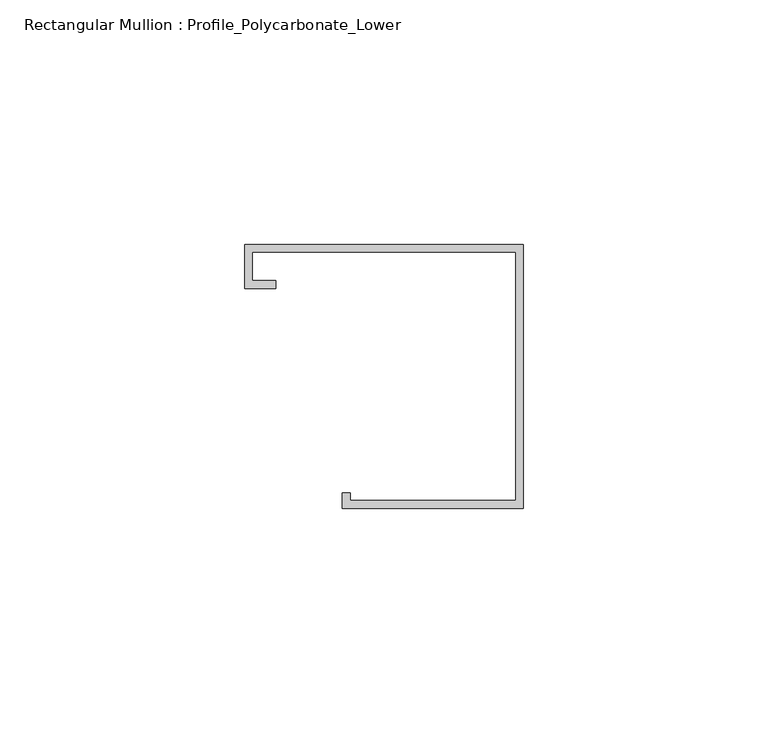
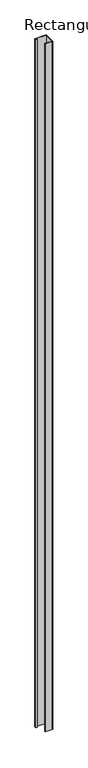
"""IFC4 building model written with IfcOpenShell, lengths in millimetres: member geometry, Rectangular Mullion : Profile_Polycarbonate_Lower."""

from ifc_helpers import new_model, si_unit, frame, origin, place, context, project, spatial, polyline, outline, extrude, source, transform, mapped, element, save


def rectangular_mullion_profile_polycarbonate_lower_0c87a6bc(model_context):
    return source(origin(), model_context, "Body", "SweptSolid", [
        extrude(outline(polyline([(0.0, 28.984575), (0.0, -25.015825), (-36.9824, -25.015825), (-36.9824, -21.840825), (-35.3949, -21.840825), (-35.3949, -23.428325), (-1.5875, -23.428325), (-1.5875, 27.397075), (-55.4101, 27.397075), (-55.4101, 21.580475), (-50.6476, 21.580475), (-50.6476, 19.992975), (-56.9976, 19.992975), (-56.9976, 28.984575), (0.0, 28.984575)])), frame((0.0, 0.0, -3626.268465), z_axis=(0.0, 0.0, 1.0), x_axis=(1.0, 0.0, 0.0)), (0.0, 0.0, 1.0), 3626.268465),
    ])


if __name__ == "__main__":
    model = new_model("IFC4")
    model_context = context("Model", 3, world=origin())
    ifc_project = project(units=[si_unit("LENGTHUNIT", "METRE", prefix="MILLI")], contexts=[model_context])
    site = spatial("IfcSite", under=ifc_project)
    building = spatial("IfcBuilding", under=site)
    placement = place(None, origin())
    rectangular_mullion_profile_polycarbonate_lower_shape = rectangular_mullion_profile_polycarbonate_lower_0c87a6bc(model_context)
    element("IfcMember", 1, ObjectType="Rectangular Mullion : Profile_Polycarbonate_Lower", at=placement, inside=building, context=model_context, shape_type="MappedRepresentation", body=[
        mapped(rectangular_mullion_profile_polycarbonate_lower_shape, transform((0.0, 0.0, 0.0), x_axis=(1.0, 0.0, 0.0), y_axis=(0.0, 1.0, 0.0), z_axis=(0.0, 0.0, 1.0))),
    ])
    save(model, "model.ifc")

# Revit data of these elements
# Type "Rectangular Mullion : Profile_Polycarbonate_Lower"
#   built-in parameter 1007322 = 0.177167 (stored number, unit not read)
#   built-in parameter 1007321 = 0 (stored number, unit not read)
#   built-in parameter 1007320 = 0.00520833 (stored number, unit not read)
